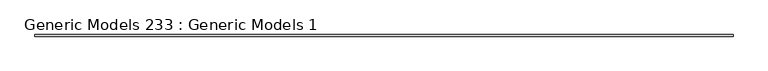
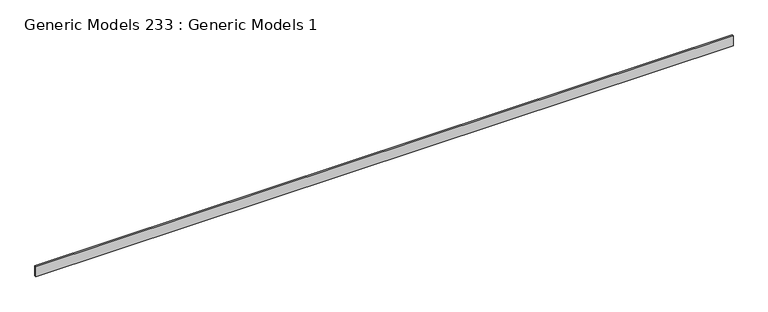
"""IFC4 building model written with IfcOpenShell, lengths in millimetres: proxy geometry, Generic Models 233 : Generic Models 1."""

from ifc_helpers import new_model, si_unit, frame, origin, place, context, project, spatial, polyline, outline, extrude, source, transform, mapped, element, save


def generic_models_233_generic_models_1_746c2673(model_context):
    return source(origin(), model_context, "Body", "SweptSolid", [
        extrude(outline(polyline([(-20998.9733045, -29227.3235041), (-20998.9733045, -29182.8735041), (-1948.9733045, -29182.8735041), (-1948.9733045, -29227.3235041), (-20998.9733045, -29227.3235041)])), frame((0.0, 0.0, 126523.496), z_axis=(0.0, 0.0, 1.0), x_axis=(1.0, 0.0, 0.0)), (0.0, 0.0, 1.0), 285.75),
    ])


if __name__ == "__main__":
    model = new_model("IFC4")
    model_context = context("Model", 3, world=origin())
    ifc_project = project(units=[si_unit("LENGTHUNIT", "METRE", prefix="MILLI")], contexts=[model_context])
    site = spatial("IfcSite", under=ifc_project)
    building = spatial("IfcBuilding", under=site)
    placement = place(None, origin())
    generic_models_233_generic_models_1_shape = generic_models_233_generic_models_1_746c2673(model_context)
    element("IfcBuildingElementProxy", 1, Name="Generic Models 233 : Generic Models 1", ObjectType="Generic Models 233 : Generic Models 1", at=placement, inside=building, context=model_context, shape_type="MappedRepresentation", body=[
        mapped(generic_models_233_generic_models_1_shape, transform((0.0, 0.0, 0.0), x_axis=(1.0, 0.0, 0.0), y_axis=(0.0, 1.0, 0.0), z_axis=(0.0, 0.0, 1.0))),
    ])
    save(model, "model.ifc")

# Revit data of these elements
# Element 1 (IfcBuildingElementProxy, "Generic Models 233 : Generic Models 1")
#   Materials on its faces: "_STRUCTURAL MEMBER (SEE STRUCT. DWGS)"
# Materials
#   "_STRUCTURAL MEMBER (SEE STRUCT. DWGS)": class "Generic", colour RGB 209 182 141, transparency 0, Cost = 0
